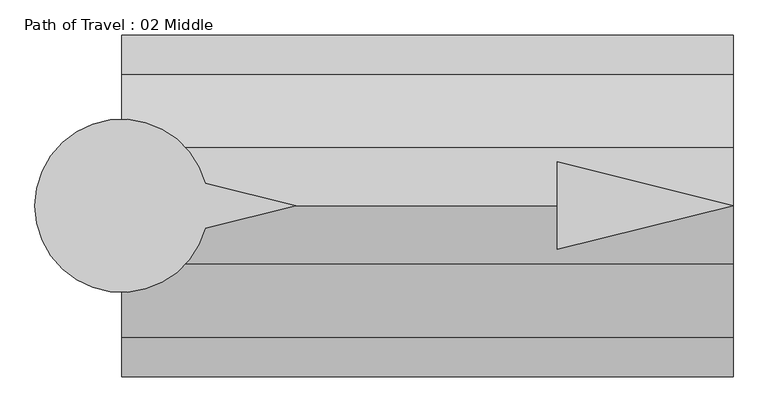
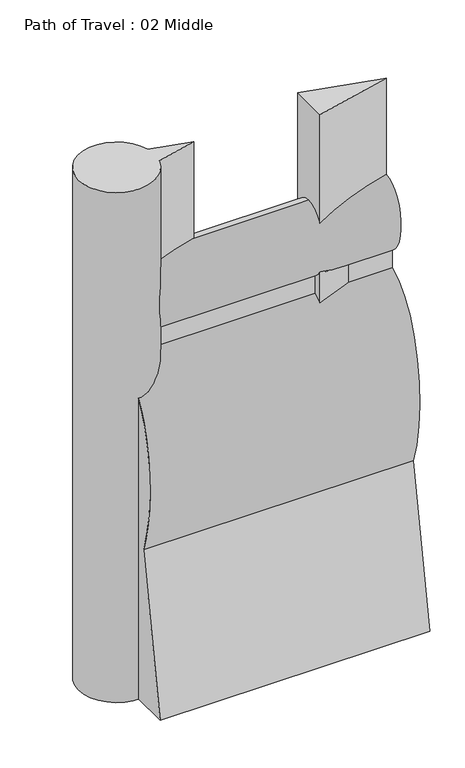
"""IFC4 building model written with IfcOpenShell, lengths in millimetres: proxy geometry, Path of Travel : 02 Middle."""

from ifc_helpers import new_model, si_unit, point, frame, frame_2d, origin, origin_with_axes, place, context, project, spatial, polyline, circle_curve, ellipse_curve, trimmed, segment, composite_curve, outline, extrude, source, transform, mapped, element, save
from ifc_brep_helpers import plane_surface, extruded_surface, advanced_brep


def path_of_travel_02_middle_8c791d19(model_context):
    return source(origin(), model_context, "Body", "SolidModel", [
        advanced_brep(
        [(227.5554837, 0.0, 1727.2), (227.5554837, 42.9018657, 1436.6534209), (227.5554837, 42.9018657, 1363.4763406), (227.5554837, 184.1186263, 643.4144547), (227.5554837, 297.5699544, 0.0), (227.5554837, 145.6574193, 0.0), (227.5554837, 0.0, 584.2), (227.5554837, -145.6574193, 0.0), (227.5554837, -297.5699544, 0.0), (227.5554837, -184.1186263, 643.4144547), (227.5554837, -42.9018657, 1363.4763406), (227.5554837, -42.9018657, 1436.6534209), (1292.5605134, 0.0, 1727.2), (1292.5605134, -42.9018657, 1436.6534209), (1292.5605134, -42.9018657, 1363.4763406), (1292.5605134, -184.1186263, 643.4144547), (1292.5605134, -297.5699544, 0.0), (1292.5605134, -145.6574193, 0.0), (1292.5605134, 0.0, 584.2), (1292.5605134, 145.6574193, 0.0), (1292.5605134, 297.5699544, 0.0), (1292.5605134, 184.1186263, 643.4144547), (1292.5605134, 42.9018657, 1363.4763406), (1292.5605134, 42.9018657, 1436.6534209)],
        [
            (0, 1, ellipse_curve(frame((227.5554837, 0.0, 1574.8), z_axis=(-1.0, 0.0, 0.0), x_axis=(0.0, 0.0, 1.0)), 152.4, 101.6)),
            (1, 2),
            (2, 3, ellipse_curve(frame((227.5554837, 0.0, 914.4), z_axis=(-1.0, 0.0, 0.0), x_axis=(0.0, 0.0, -1.0)), 457.2, 228.6)),
            (3, 4),
            (4, 5),
            (5, 6),
            (6, 7),
            (7, 8),
            (8, 9),
            (9, 10, ellipse_curve(frame((227.5554837, 0.0, 914.4), z_axis=(-1.0, 0.0, 0.0), x_axis=(0.0, 0.0, -1.0)), 457.2, 228.6)),
            (10, 11),
            (11, 0, ellipse_curve(frame((227.5554837, 0.0, 1574.8), z_axis=(-1.0, 0.0, 0.0), x_axis=(0.0, 0.0, 1.0)), 152.4, 101.6)),
            (12, 13, ellipse_curve(frame((1292.5605134, 0.0, 1574.8), z_axis=(1.0, 0.0, 0.0), x_axis=(0.0, 0.0, 1.0)), 152.4, 101.6)),
            (13, 14),
            (14, 15, ellipse_curve(frame((1292.5605134, 0.0, 914.4), z_axis=(1.0, 0.0, 0.0), x_axis=(0.0, 0.0, -1.0)), 457.2, 228.6)),
            (15, 16),
            (16, 17),
            (17, 18),
            (18, 19),
            (19, 20),
            (20, 21),
            (21, 22, ellipse_curve(frame((1292.5605134, 0.0, 914.4), z_axis=(1.0, 0.0, 0.0), x_axis=(0.0, 0.0, -1.0)), 457.2, 228.6)),
            (22, 23),
            (23, 12, ellipse_curve(frame((1292.5605134, 0.0, 1574.8), z_axis=(1.0, 0.0, 0.0), x_axis=(0.0, 0.0, 1.0)), 152.4, 101.6)),
            (0, 12),
            (23, 1),
            (22, 2),
            (21, 3),
            (20, 4),
            (19, 5),
            (18, 6),
            (17, 7),
            (16, 8),
            (15, 9),
            (14, 10),
            (13, 11),
        ],
        [
            plane_surface(frame((227.5554837, 0.0, 0.0), z_axis=(-1.0, 0.0, 0.0), x_axis=(0.0, 0.0, 1.0))),
            plane_surface(frame((1292.5605134, 0.0, 0.0), z_axis=(1.0, 0.0, 0.0), x_axis=(0.0, 0.0, 1.0))),
            extruded_surface(trimmed(ellipse_curve(frame((1292.5605134, 0.0, 1574.8), z_axis=(-1.0, 0.0, 0.0), x_axis=(0.0, 0.0, 1.0)), 152.4, 101.6), [point((1292.5605134, 0.0, 1727.2))], [point((1292.5605134, 42.9018657, 1436.6534209))], True, "CARTESIAN"), (-1065.0050297, 0.0, 0.0), 1065.0050297),
            plane_surface(frame((227.5554837, 42.9018657, 1436.6534209), z_axis=(0.0, 1.0, 0.0), x_axis=(1.0, 0.0, 0.0))),
            extruded_surface(trimmed(ellipse_curve(frame((1292.5605134, 0.0, 914.4), z_axis=(-1.0, 0.0, 0.0), x_axis=(0.0, 0.0, -1.0)), 457.2, 228.6), [point((1292.5605134, 42.9018657, 1363.4763406))], [point((1292.5605134, 184.1186263, 643.4144547))], True, "CARTESIAN"), (-1065.0050297, 0.0, 0.0), 1065.0050297),
            plane_surface(frame((227.5554837, 184.1186263, 643.4144547), z_axis=(0.0, 0.9848077530122078, 0.1736481776669322), x_axis=(1.0, 0.0, 0.0))),
            plane_surface(frame((227.5554837, 297.5699544, 0.0), z_axis=(0.0, 0.0, -1.0), x_axis=(1.0, 0.0, 0.0))),
            plane_surface(frame((227.5554837, 145.6574193, 0.0), z_axis=(0.0, -0.9702957262760199, -0.2419218955995739), x_axis=(1.0, 0.0, 0.0))),
            plane_surface(frame((227.5554837, 0.0, 584.2), z_axis=(0.0, 0.9702957262759961, -0.24192189559966923), x_axis=(1.0, 0.0, 0.0))),
            plane_surface(frame((227.5554837, -145.6574193, 0.0), z_axis=(0.0, 0.0, -1.0), x_axis=(1.0, 0.0, 0.0))),
            plane_surface(frame((227.5554837, -297.5699544, 0.0), z_axis=(0.0, -0.984807753012208, 0.17364817766693066), x_axis=(1.0, 0.0, 0.0))),
            extruded_surface(trimmed(ellipse_curve(frame((1292.5605134, 0.0, 914.4), z_axis=(-1.0, 0.0, 0.0), x_axis=(0.0, 0.0, -1.0)), 457.2, 228.6), [point((1292.5605134, -184.1186263, 643.4144547))], [point((1292.5605134, -42.9018657, 1363.4763406))], True, "CARTESIAN"), (-1065.0050297, 0.0, 0.0), 1065.0050297),
            plane_surface(frame((227.5554837, -42.9018657, 1363.4763406), z_axis=(0.0, -1.0, 0.0), x_axis=(1.0, 0.0, 0.0))),
            extruded_surface(trimmed(ellipse_curve(frame((1292.5605134, 0.0, 1574.8), z_axis=(-1.0, 0.0, 0.0), x_axis=(0.0, 0.0, 1.0)), 152.4, 101.6), [point((1292.5605134, -42.9018657, 1436.6534209))], [point((1292.5605134, 0.0, 1727.2))], True, "CARTESIAN"), (-1065.0050297, 0.0, 0.0), 1065.0050297),
        ],
        [
            (0, [[1, 2, 3, 4, 5, 6, 7, 8, 9, 10, 11, 12]]),
            (1, [[13, 14, 15, 16, 17, 18, 19, 20, 21, 22, 23, 24]]),
            (2, [[-1, 25, -24, 26]]),
            (3, [[-2, -26, -23, 27]]),
            (4, [[-3, -27, -22, 28]]),
            (5, [[-4, -28, -21, 29]]),
            (6, [[-5, -29, -20, 30]]),
            (7, [[-6, -30, -19, 31]]),
            (8, [[-7, -31, -18, 32]]),
            (9, [[-8, -32, -17, 33]]),
            (10, [[-9, -33, -16, 34]]),
            (11, [[-10, -34, -15, 35]]),
            (12, [[-11, -35, -14, 36]]),
            (13, [[-12, -36, -13, -25]]),
        ],
    ),
        extrude(outline(polyline([(986.5553669, 76.2006338), (1292.5605134, 0.0), (986.5553669, -76.2006338), (986.5553669, 76.2006338)])), origin_with_axes(), (0.0, 0.0, 1.0), 2129.5973753),
        extrude(outline(composite_curve([segment(polyline([(372.7837828, 39.4440225), (531.182385, 0.0), (372.7837828, -39.4440225)]), True, "CONTINUOUS"), segment(trimmed(circle_curve(frame_2d((227.2200886, 0.0)), 150.8131956), [point((372.7837828, -39.4440225))], [point((372.7837828, 39.4440225))], False, "CARTESIAN"), True, "CONTINUOUS")], self_intersect=False)), origin_with_axes(), (0.0, 0.0, 1.0), 2129.5973753),
    ])


if __name__ == "__main__":
    model = new_model("IFC4")
    model_context = context("Model", 3, world=origin())
    ifc_project = project(units=[si_unit("LENGTHUNIT", "METRE", prefix="MILLI")], contexts=[model_context])
    site = spatial("IfcSite", under=ifc_project)
    building = spatial("IfcBuilding", under=site)
    placement = place(None, origin())
    path_of_travel_02_middle_shape = path_of_travel_02_middle_8c791d19(model_context)
    element("IfcBuildingElementProxy", 1, Name="Path of Travel : 02 Middle", ObjectType="Path of Travel : 02 Middle", at=placement, inside=building, context=model_context, shape_type="MappedRepresentation", body=[
        mapped(path_of_travel_02_middle_shape, transform((0.0, 0.0, 0.0), x_axis=(1.0, 0.0, 0.0), y_axis=(0.0, 1.0, 0.0), z_axis=(0.0, 0.0, 1.0))),
    ])
    save(model, "model.ifc")

# Revit data of these elements
# Type "Path of Travel : 02 Middle"
#   Path of Egress [instance default] = 4' - 0"
#   built-in parameter 1001306 [instance default] = 4 (stored number, unit not read)
#   Dot at Start = no
#   Arrow in Middle = yes
#   Arrow at End = no
#   Egress Path = none
# Element 1 (IfcBuildingElementProxy, "Path of Travel : 02 Middle")
#   Path of Egress = 3' - 5.92933"
#   built-in parameter 1001306 = 3.49411 (stored number, unit not read)
#   Materials on its faces: "Egress Path Solid", "solid"
# Materials
#   "Egress Path Solid": class "Unassigned", colour RGB 255 128 64, transparency 0.75, Comments = "Rendering appearance not upgraded "
#   "solid": class "Generic", colour RGB 120 120 120, transparency 0, Cost = 0
